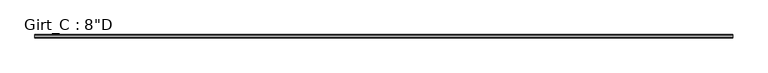
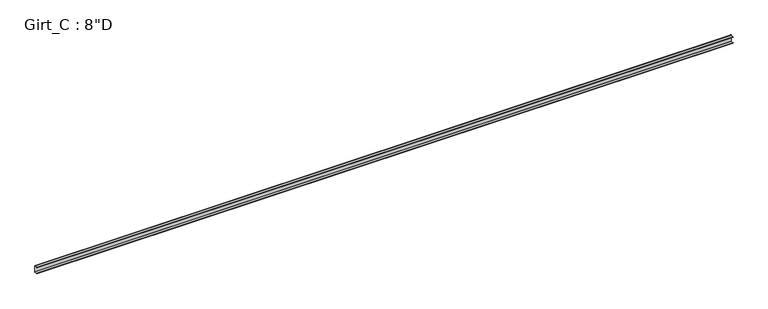
"""IFC4 building model written with IfcOpenShell, lengths in millimetres: beam geometry."""

from ifc_helpers import new_model, si_unit, point, frame, frame_2d, origin, place, context, project, spatial, polyline, circle_curve, trimmed, segment, composite_curve, outline, extrude, source, transform, mapped, element, save


def beam_f53cf365(model_context):
    return source(origin(), model_context, "Body", "SweptSolid", [
        extrude(outline(composite_curve([segment(polyline([(-87.5109375, 101.6), (-3.3734375, 101.6)]), True, "CONTINUOUS"), segment(trimmed(circle_curve(frame_2d((-3.3734375, 96.8375)), 4.7625), [point((-3.3734375, 101.6))], [point((1.3890625, 96.8375))], False, "CARTESIAN"), True, "CONTINUOUS"), segment(polyline([(1.3890625, 96.8375), (1.3890625, -96.8375)]), True, "CONTINUOUS"), segment(trimmed(circle_curve(frame_2d((-3.3734375, -96.8375)), 4.7625), [point((1.3890625, -96.8375))], [point((-3.3734375, -101.6))], False, "CARTESIAN"), True, "CONTINUOUS"), segment(polyline([(-3.3734375, -101.6), (-87.5109375, -101.6), (-99.7792647, -86.979177), (-97.6510975, -85.1934327), (-86.2154765, -98.821875), (-3.2694106, -98.821875)]), True, "CONTINUOUS"), segment(trimmed(circle_curve(frame_2d((-3.3748024, -96.8389339)), 1.9857399), [point((-3.2694106, -98.821875))], [point((-1.3890625, -96.8389339))], True, "CARTESIAN"), True, "CONTINUOUS"), segment(polyline([(-1.3890625, -96.8389339), (-1.3890625, 96.8381931)]), True, "CONTINUOUS"), segment(trimmed(circle_curve(frame_2d((-3.3741066, 96.8381931)), 1.9850441), [point((-1.3890625, 96.8381931))], [point((-3.3005807, 98.821875))], True, "CARTESIAN"), True, "CONTINUOUS"), segment(polyline([(-3.3005807, 98.821875), (-86.2154765, 98.821875), (-97.6278742, 85.221109), (-99.7560415, 87.0068534), (-87.5109375, 101.6)]), True, "CONTINUOUS")], self_intersect=False)), frame((-10301.2875, 0.0, 0.0), z_axis=(1.0, 0.0, 0.0), x_axis=(0.0, 1.0, 0.0)), (0.0, 0.0, 1.0), 20657.439),
    ])


if __name__ == "__main__":
    model = new_model("IFC4")
    model_context = context("Model", 3, world=origin())
    ifc_project = project(units=[si_unit("LENGTHUNIT", "METRE", prefix="MILLI")], contexts=[model_context])
    site = spatial("IfcSite", under=ifc_project)
    building = spatial("IfcBuilding", under=site)
    placement = place(None, origin())
    beam_shape = beam_f53cf365(model_context)
    element("IfcBeam", 1, ObjectType="Girt_C : 8\"D", at=placement, inside=building, context=model_context, shape_type="MappedRepresentation", body=[
        mapped(beam_shape, transform((0.0, 0.0, 0.0), x_axis=(1.0, 0.0, 0.0), y_axis=(0.0, 1.0, 0.0), z_axis=(0.0, 0.0, 1.0))),
    ])
    save(model, "model.ifc")

# Revit data of these elements
# Type "Girt_C : 8\"D"
#   half leg = 0' - 1 3/4"
#   Web_Thickness = 0' - 0 7/64"
#   Length [instance default] = 10' - 0"
#   Leg_1 = 0' - 3 1/2"
#   Height = 0' - 8"
#   Structural Material [instance default] = none
# Element 1 (IfcBeam, "Girt_C : 8\"D")
#   Structural Material = CEE' SECTION (8.0x3.5C - SEE STRUCT. DWGS)
#   Materials on its faces: "CEE' SECTION (8.0x3.5C - SEE STRUCT. DWGS)"
# Materials
#   "CEE' SECTION (8.0x3.5C - SEE STRUCT. DWGS)": class "Metal", colour RGB 137 146 153, transparency 0, Description = "Steel, mill finish", Cost = 0
